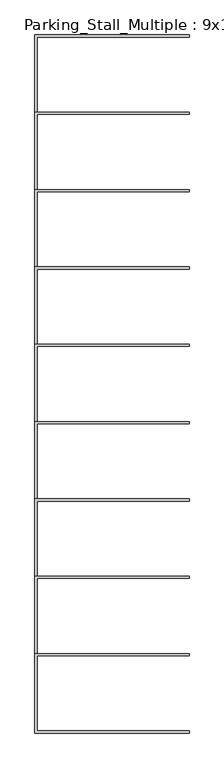
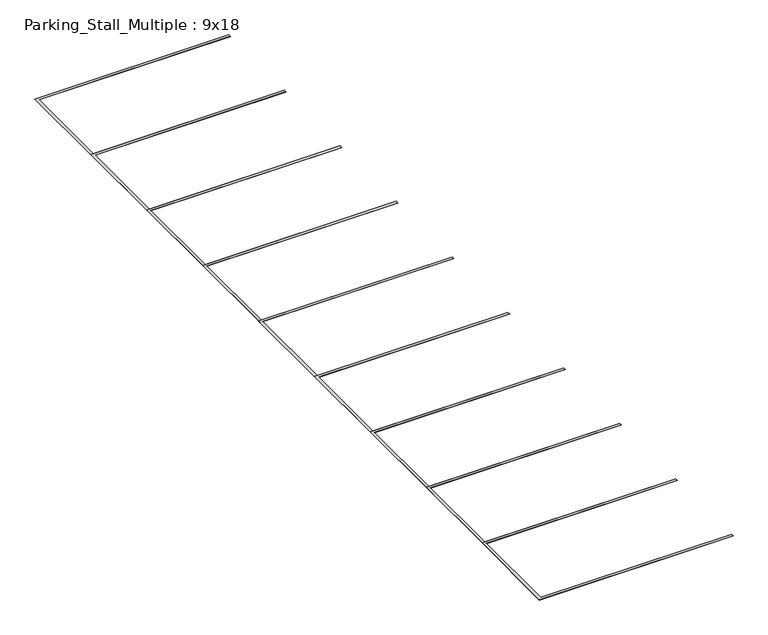
"""IFC4 building model written with IfcOpenShell, lengths in millimetres: proxy geometry, Parking_Stall_Multiple : 9x18."""

from ifc_helpers import new_model, si_unit, origin, origin_with_axes, place, context, project, spatial, polyline, outline, extrude, source, transform, mapped, element, save


def parking_stall_multiple_9x18_3a9ea78d(model_context):
    return source(origin(), model_context, "Body", "SweptSolid", [
        extrude(outline(polyline([(5486.4, -21945.6), (5486.4, -22021.8), (76.2, -22021.8), (76.2, -24688.8), (5486.4, -24688.8), (5486.4, -24765.0), (0.0, -24765.0), (0.0, -21945.6), (5486.4, -21945.6)])), origin_with_axes(), (0.0, 0.0, 1.0), 6.35),
        extrude(outline(polyline([(5486.4, -19202.4), (5486.4, -19278.6), (76.2, -19278.6), (76.2, -21945.6), (5486.4, -21945.6), (5486.4, -22021.8), (0.0, -22021.8), (0.0, -19202.4), (5486.4, -19202.4)])), origin_with_axes(), (0.0, 0.0, 1.0), 6.35),
        extrude(outline(polyline([(5486.4, -16459.2), (5486.4, -16535.4), (76.2, -16535.4), (76.2, -19202.4), (5486.4, -19202.4), (5486.4, -19278.6), (0.0, -19278.6), (0.0, -16459.2), (5486.4, -16459.2)])), origin_with_axes(), (0.0, 0.0, 1.0), 6.35),
        extrude(outline(polyline([(5486.4, -13716.0), (5486.4, -13792.2), (76.2, -13792.2), (76.2, -16459.2), (5486.4, -16459.2), (5486.4, -16535.4), (0.0, -16535.4), (0.0, -13716.0), (5486.4, -13716.0)])), origin_with_axes(), (0.0, 0.0, 1.0), 6.35),
        extrude(outline(polyline([(5486.4, -10972.8), (5486.4, -11049.0), (76.2, -11049.0), (76.2, -13716.0), (5486.4, -13716.0), (5486.4, -13792.2), (0.0, -13792.2), (0.0, -10972.8), (5486.4, -10972.8)])), origin_with_axes(), (0.0, 0.0, 1.0), 6.35),
        extrude(outline(polyline([(5486.4, -8229.6), (5486.4, -8305.8), (76.2, -8305.8), (76.2, -10972.8), (5486.4, -10972.8), (5486.4, -11049.0), (0.0, -11049.0), (0.0, -8229.6), (5486.4, -8229.6)])), origin_with_axes(), (0.0, 0.0, 1.0), 6.35),
        extrude(outline(polyline([(5486.4, -5486.4), (5486.4, -5562.6), (76.2, -5562.6), (76.2, -8229.6), (5486.4, -8229.6), (5486.4, -8305.8), (0.0, -8305.8), (0.0, -5486.4), (5486.4, -5486.4)])), origin_with_axes(), (0.0, 0.0, 1.0), 6.35),
        extrude(outline(polyline([(5486.4, -2743.2), (5486.4, -2819.4), (76.2, -2819.4), (76.2, -5486.4), (5486.4, -5486.4), (5486.4, -5562.6), (0.0, -5562.6), (0.0, -2743.2), (5486.4, -2743.2)])), origin_with_axes(), (0.0, 0.0, 1.0), 6.35),
        extrude(outline(polyline([(5486.4, 0.0), (5486.4, -76.2), (76.2, -76.2), (76.2, -2743.2), (5486.4, -2743.2), (5486.4, -2819.4), (0.0, -2819.4), (0.0, 0.0), (5486.4, 0.0)])), origin_with_axes(), (0.0, 0.0, 1.0), 6.35),
    ])


if __name__ == "__main__":
    model = new_model("IFC4")
    model_context = context("Model", 3, world=origin())
    ifc_project = project(units=[si_unit("LENGTHUNIT", "METRE", prefix="MILLI")], contexts=[model_context])
    site = spatial("IfcSite", under=ifc_project)
    building = spatial("IfcBuilding", under=site)
    placement = place(None, origin())
    parking_stall_multiple_9x18_shape = parking_stall_multiple_9x18_3a9ea78d(model_context)
    element("IfcBuildingElementProxy", 1, Name="Parking_Stall_Multiple : 9x18", ObjectType="Parking_Stall_Multiple : 9x18", at=placement, inside=building, context=model_context, shape_type="MappedRepresentation", body=[
        mapped(parking_stall_multiple_9x18_shape, transform((0.0, 0.0, 0.0), x_axis=(1.0, 0.0, 0.0), y_axis=(0.0, 1.0, 0.0), z_axis=(0.0, 0.0, 1.0))),
    ])
    save(model, "model.ifc")

# Revit data of these elements
# Type "Parking_Stall_Multiple : 9x18"
#   Parking_Width_M = 9' - 0"
#   Parking_Run_Length [instance default] = 65' - 0"
#   Parking_Line_Width = 0' - 3"
#   Parking_Length_M = 18' - 0"
#   Single_Parking_Visibility [instance default] = no
#   Parking_ADA_Symbol = no
#   ParkingUnitsArray [instance default] = 7
#   ParkingUnits [instance default] = 7
#   Multiple_Parking_Visibility [instance default] = yes
#   Parking_Line_Material = none
# Element 1 (IfcBuildingElementProxy, "Parking_Stall_Multiple : 9x18")
#   Parking_Run_Length = 81' - 3"
#   ParkingUnitsArray = 9
#   ParkingUnits = 9
